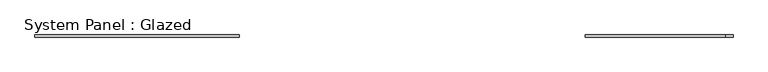
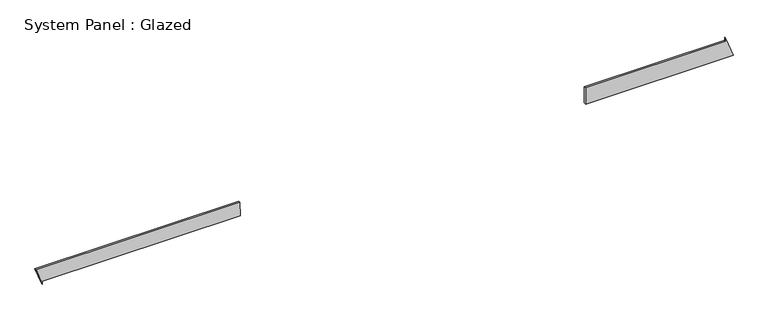
"""IFC4 building model written with IfcOpenShell, lengths in millimetres: plate geometry, System Panel : Glazed."""

import ifcopenshell
import ifcopenshell.guid

model = None  # the IFC model being written
_history = None  # IfcOwnerHistory: only IFC2X3 demands one
_inside = {}  # id of a spatial element -> (the spatial element, [elements in it])
_under = {}  # id of a project, library or spatial element -> (it, [spatial elements below it])
_declared = {}  # id of a project -> (the project, [libraries it declares])
_typed = {}  # id of a type object -> (the type object, [elements of that type])
_made_of = {}  # id of a material, layer set ... -> (it, [elements and type objects made of it])


def new_model(schema):
    """Start an empty IFC model of exactly this schema.

    Asked for "IFC4X3", IfcOpenShell would pick the latest addendum, in which some entities
    have other attributes; the version numbers below select the first issue.
    IFC2X3 requires an IfcOwnerHistory on every rooted entity: one is made here for all.
    """
    global model, _history
    if schema == "IFC4X3":
        model = ifcopenshell.file(schema_version=(4, 3, 0, 0))
    else:
        model = ifcopenshell.file(schema=schema)
    _inside.clear()
    _under.clear()
    _declared.clear()
    _typed.clear()
    _made_of.clear()
    _history = None
    if model.schema == "IFC2X3":
        org = make("IfcOrganization", Name="unknown")
        user = make(
            "IfcPersonAndOrganization",
            ThePerson=make("IfcPerson", FamilyName="unknown"),
            TheOrganization=org,
        )
        app = make(
            "IfcApplication",
            ApplicationDeveloper=org,
            Version="unknown",
            ApplicationFullName="unknown",
            ApplicationIdentifier="unknown",
        )
        _history = make(
            "IfcOwnerHistory",
            OwningUser=user,
            OwningApplication=app,
            ChangeAction="ADDED",
            CreationDate=0,
        )
    return model


def make(cls, **values):
    """One entity of the class cls with the attributes given. An attribute that is None is left unset."""
    return model.create_entity(
        cls, **{name: value for name, value in values.items() if value is not None}
    )


def rooted(cls, **values):
    """An entity with a GlobalId (a new one), such as an element, a storey or a relation."""
    return make(cls, GlobalId=ifcopenshell.guid.new(), OwnerHistory=_history, **values)


def si_unit(unit_type, name, prefix=None):
    """IfcSIUnit, for example si_unit("LENGTHUNIT", "METRE", prefix="MILLI")."""
    return make("IfcSIUnit", UnitType=unit_type, Prefix=prefix, Name=name)


def assignment(units):
    """IfcUnitAssignment: the units of a project."""
    return None if units is None else make("IfcUnitAssignment", Units=units)


def point(xyz):
    """IfcCartesianPoint."""
    return None if xyz is None else make("IfcCartesianPoint", Coordinates=xyz)


def direction(xyz):
    """IfcDirection."""
    return None if xyz is None else make("IfcDirection", DirectionRatios=xyz)


def frame(location, z_axis=None, x_axis=None):
    """IfcAxis2Placement3D, a coordinate frame: its origin and axes. An axis left out is left unset."""
    return make(
        "IfcAxis2Placement3D",
        Location=point(location),
        Axis=direction(z_axis),
        RefDirection=direction(x_axis),
    )


def origin():
    """The frame at (0, 0, 0) with its axes left unset."""
    return frame((0.0, 0.0, 0.0))


def place(relative_to, where):
    """IfcLocalPlacement: puts the frame where relative to a parent placement (None: the world)."""
    return make(
        "IfcLocalPlacement", PlacementRelTo=relative_to, RelativePlacement=where
    )


def context(
    kind, dimensions, precision=None, world=None, true_north=None, identifier=None
):
    """IfcGeometricRepresentationContext, for example the 3D "Model" context."""
    return make(
        "IfcGeometricRepresentationContext",
        ContextIdentifier=identifier,
        ContextType=kind,
        CoordinateSpaceDimension=dimensions,
        Precision=precision,
        WorldCoordinateSystem=world,
        TrueNorth=true_north,
    )


def project(units=None, contexts=None):
    """IfcProject with its units and contexts."""
    return rooted(
        "IfcProject",
        Name="project",
        RepresentationContexts=contexts,
        UnitsInContext=assignment(units),
    )


def spatial(cls, under=None, at=None, **own):
    """A site, building, storey or space (cls), placed at a placement, below another one or the project."""
    s = rooted(cls, ObjectPlacement=at, **own)
    if under is not None:
        _under.setdefault(under.id(), (under, []))[1].append(s)
    return s


def polyline(points):
    """IfcPolyline through the points."""
    return make("IfcPolyline", Points=[point(p) for p in points])


def outline(outer, holes=None, kind="AREA"):
    """IfcArbitraryClosedProfileDef: a profile drawn as a closed curve; with holes, ...WithVoids."""
    if holes is None:
        return make("IfcArbitraryClosedProfileDef", ProfileType=kind, OuterCurve=outer)
    return make(
        "IfcArbitraryProfileDefWithVoids",
        ProfileType=kind,
        OuterCurve=outer,
        InnerCurves=holes,
    )


def extrude(swept, where, along, depth):
    """IfcExtrudedAreaSolid: the profile swept, set in the frame where, extruded along a direction by depth."""
    return make(
        "IfcExtrudedAreaSolid",
        SweptArea=swept,
        Position=where,
        ExtrudedDirection=direction(along),
        Depth=depth,
    )


def shape(context_of_items, identifier, shape_type, items):
    """IfcShapeRepresentation: the items that make up one representation, for example the "Body"."""
    return make(
        "IfcShapeRepresentation",
        ContextOfItems=context_of_items,
        RepresentationIdentifier=identifier,
        RepresentationType=shape_type,
        Items=items,
    )


def source(mapping_origin, context_of_items, identifier, shape_type, items):
    """IfcRepresentationMap: a shape defined once, which mapped items show again and again."""
    return make(
        "IfcRepresentationMap",
        MappingOrigin=mapping_origin,
        MappedRepresentation=shape(context_of_items, identifier, shape_type, items),
    )


def transform(
    local_origin,
    x_axis=None,
    y_axis=None,
    z_axis=None,
    scale=None,
    scale2=None,
    scale3=None,
    uniform=True,
):
    """IfcCartesianTransformationOperator3D, or its non-uniform kind. x_axis, y_axis, z_axis: its Axis1, 2, 3."""
    if uniform:
        return make(
            "IfcCartesianTransformationOperator3D",
            Axis1=direction(x_axis),
            Axis2=direction(y_axis),
            LocalOrigin=point(local_origin),
            Scale=scale,
            Axis3=direction(z_axis),
        )
    return make(
        "IfcCartesianTransformationOperator3DnonUniform",
        Axis1=direction(x_axis),
        Axis2=direction(y_axis),
        LocalOrigin=point(local_origin),
        Scale=scale,
        Axis3=direction(z_axis),
        Scale2=scale2,
        Scale3=scale3,
    )


def mapped(mapping_source, mapping_target):
    """IfcMappedItem: shows the shape of a source again, moved by a transform."""
    return make(
        "IfcMappedItem", MappingSource=mapping_source, MappingTarget=mapping_target
    )


def made_of(thing, what):
    """Note that an element or type object is made of a material, layer set ...; save() writes the relation."""
    if what is not None:
        _made_of.setdefault(what.id(), (what, []))[1].append(thing)
    return thing


def element(
    cls,
    number,
    at=None,
    inside=None,
    cuts=None,
    type_object=None,
    material=None,
    context=None,
    identifier="Body",
    shape_type=None,
    held_by="IfcProductDefinitionShape",
    body=None,
    shapes=None,
    **own,
):
    """One element of the class cls, such as IfcWall. Its Tag is "e" and its number.

    at: its placement. inside: the storey or other place that contains it. cuts: it is an
    opening in that element (IfcRelVoidsElement). A single representation is given by context,
    identifier, shape_type and body (its items); several are given by shapes. held_by: the class
    of the entity that holds the representations. save() writes the other relations.
    """
    e = rooted(cls, Tag="e%d" % number, ObjectPlacement=at, **own)
    if body is not None:
        shapes = [shape(context, identifier, shape_type, body)]
    if shapes is not None:
        e.Representation = make(held_by, Representations=shapes)
    if inside is not None:
        _inside.setdefault(inside.id(), (inside, []))[1].append(e)
    if cuts is not None:
        rooted(
            "IfcRelVoidsElement", RelatingBuildingElement=cuts, RelatedOpeningElement=e
        )
    if type_object is not None:
        _typed.setdefault(type_object.id(), (type_object, []))[1].append(e)
    return made_of(e, material)


def aggregate(whole, parts):
    """IfcRelAggregates: a whole, such as a stair, and the parts it consists of."""
    return rooted("IfcRelAggregates", RelatingObject=whole, RelatedObjects=parts)


def save(model, path):
    """Write the relations noted so far, then the file.

    IfcRelAggregates (storeys below a building ...), IfcRelContainedInSpatialStructure (elements
    in a storey), IfcRelDefinesByType, IfcRelAssociatesMaterial and IfcRelDeclares: one each for
    every whole, place, type object, material and project.
    """
    for whole, parts in _under.values():
        aggregate(whole, parts)
    for where, things in _inside.values():
        rooted(
            "IfcRelContainedInSpatialStructure",
            RelatedElements=things,
            RelatingStructure=where,
        )
    for kind, things in _typed.values():
        rooted("IfcRelDefinesByType", RelatedObjects=things, RelatingType=kind)
    for what, things in _made_of.values():
        rooted("IfcRelAssociatesMaterial", RelatedObjects=things, RelatingMaterial=what)
    for by, libraries in _declared.values():
        rooted("IfcRelDeclares", RelatingContext=by, RelatedDefinitions=libraries)
    model.write(path)


def system_panel_glazed_c0f42e98(model_context):
    return source(origin(), model_context, "Body", "SweptSolid", [
        extrude(outline(polyline([(0.0, 2327.1115757), (0.0, 4034.6007191), (234.3998836, 3949.9537418), (199.0445445, 3949.9522175), (199.114455, 2328.4254713), (0.0, 2327.1115757)])), frame((0.0, -49.5, 0.0), z_axis=(0.0, 1.0, 0.0), x_axis=(0.0, 0.0, 1.0)), (0.0, 0.0, 1.0), 25.0),
        extrude(outline(polyline([(0.0, -3963.5189783), (35.3553391, -3963.5189783), (35.3553391, -1673.7284407), (199.2870376, -1674.5133491), (199.3887904, -4034.6007191), (0.0, -3963.5189783)])), frame((0.0, -49.5, 0.0), z_axis=(0.0, 1.0, 0.0), x_axis=(0.0, 0.0, 1.0)), (0.0, 0.0, 1.0), 25.0),
    ])


if __name__ == "__main__":
    model = new_model("IFC4")
    model_context = context("Model", 3, world=origin())
    ifc_project = project(units=[si_unit("LENGTHUNIT", "METRE", prefix="MILLI")], contexts=[model_context])
    site = spatial("IfcSite", under=ifc_project)
    building = spatial("IfcBuilding", under=site)
    placement = place(None, origin())
    system_panel_glazed_shape = system_panel_glazed_c0f42e98(model_context)
    element("IfcPlate", 1, ObjectType="System Panel : Glazed", at=placement, inside=building, context=model_context, shape_type="MappedRepresentation", body=[
        mapped(system_panel_glazed_shape, transform((0.0, 0.0, 0.0), x_axis=(1.0, 0.0, 0.0), y_axis=(0.0, 1.0, 0.0), z_axis=(0.0, 0.0, 1.0))),
    ])
    save(model, "model.ifc")

# Revit data of these elements
# Element 1 (IfcPlate, "System Panel : Glazed")
#   Materials on its faces: "Glass"
# Materials
#   "Glass": class "Glass", colour RGB 218 227 224, transparency 0.85, Description = "Soda Lime Glass", Cost = 0
